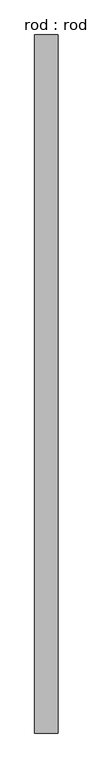
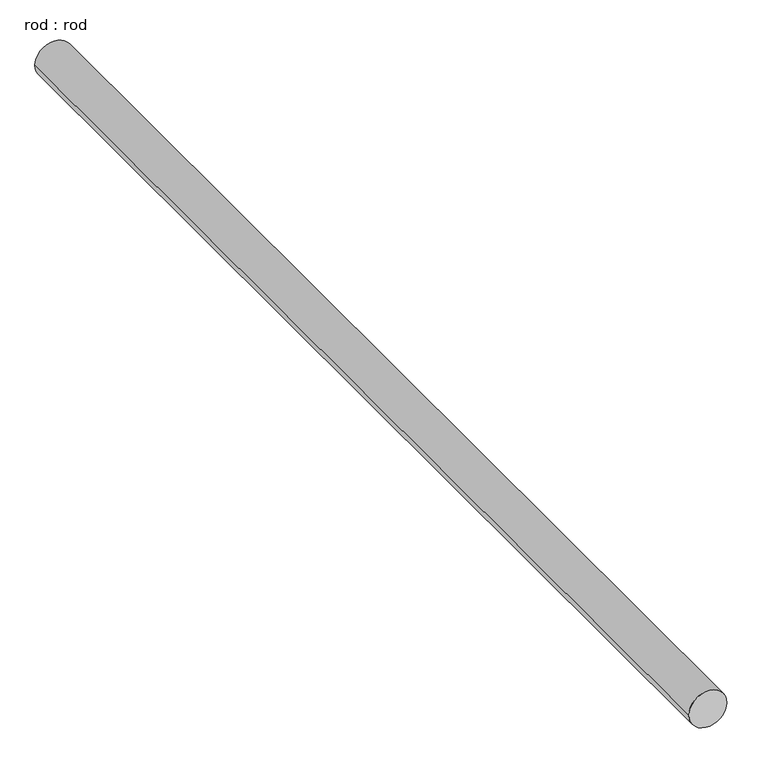
"""IFC4 building model written with IfcOpenShell, lengths in millimetres: proxy geometry, rod : rod."""

from ifc_helpers import new_model, si_unit, point, frame, frame_2d, origin, place, context, project, spatial, circle_curve, trimmed, segment, composite_curve, outline, extrude, source, transform, mapped, element, save


def rod_rod_2a650fe3(model_context):
    return source(origin(), model_context, "Body", "SweptSolid", [
        extrude(outline(composite_curve([segment(trimmed(circle_curve(frame_2d((0.0108462, 0.0)), 200.0), [point((0.0108462, 200.0))], [point((0.0108462, -200.0))], False, "CARTESIAN"), True, "CONTINUOUS"), segment(trimmed(circle_curve(frame_2d((0.0108462, 0.0)), 200.0), [point((0.0108462, -200.0))], [point((0.0108462, 200.0))], False, "CARTESIAN"), True, "CONTINUOUS")], self_intersect=False)), frame((0.0, -1867.6614726, 0.0), z_axis=(0.0, 1.0, 0.0), x_axis=(0.0, 0.0, 1.0)), (0.0, 0.0, 1.0), 11920.7801758),
    ])


if __name__ == "__main__":
    model = new_model("IFC4")
    model_context = context("Model", 3, world=origin())
    ifc_project = project(units=[si_unit("LENGTHUNIT", "METRE", prefix="MILLI")], contexts=[model_context])
    site = spatial("IfcSite", under=ifc_project)
    building = spatial("IfcBuilding", under=site)
    placement = place(None, origin())
    rod_rod_shape = rod_rod_2a650fe3(model_context)
    element("IfcBuildingElementProxy", 1, Name="rod : rod", ObjectType="rod : rod", at=placement, inside=building, context=model_context, shape_type="MappedRepresentation", body=[
        mapped(rod_rod_shape, transform((0.0, 0.0, 0.0), x_axis=(1.0, 0.0, 0.0), y_axis=(0.0, 1.0, 0.0), z_axis=(0.0, 0.0, 1.0))),
    ])
    save(model, "model.ifc")

# Revit data of these elements
# Type "rod : rod"
#   Default Elevation = 0
